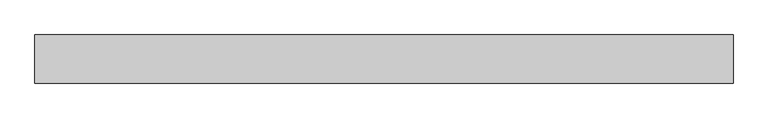
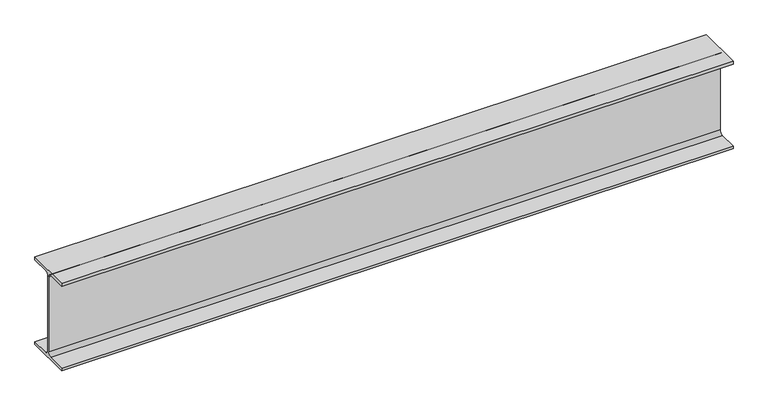
"""IFC4 building model written with IfcOpenShell, lengths in millimetres: beam geometry, 0912_Steel Framing_H-KSD3502 : H_SB_ASB_H-350x175x7x11."""

import ifcopenshell
import ifcopenshell.guid

model = None  # the IFC model being written
_history = None  # IfcOwnerHistory: only IFC2X3 demands one
_inside = {}  # id of a spatial element -> (the spatial element, [elements in it])
_under = {}  # id of a project, library or spatial element -> (it, [spatial elements below it])
_declared = {}  # id of a project -> (the project, [libraries it declares])
_typed = {}  # id of a type object -> (the type object, [elements of that type])
_made_of = {}  # id of a material, layer set ... -> (it, [elements and type objects made of it])


def new_model(schema):
    """Start an empty IFC model of exactly this schema.

    Asked for "IFC4X3", IfcOpenShell would pick the latest addendum, in which some entities
    have other attributes; the version numbers below select the first issue.
    IFC2X3 requires an IfcOwnerHistory on every rooted entity: one is made here for all.
    """
    global model, _history
    if schema == "IFC4X3":
        model = ifcopenshell.file(schema_version=(4, 3, 0, 0))
    else:
        model = ifcopenshell.file(schema=schema)
    _inside.clear()
    _under.clear()
    _declared.clear()
    _typed.clear()
    _made_of.clear()
    _history = None
    if model.schema == "IFC2X3":
        org = make("IfcOrganization", Name="unknown")
        user = make(
            "IfcPersonAndOrganization",
            ThePerson=make("IfcPerson", FamilyName="unknown"),
            TheOrganization=org,
        )
        app = make(
            "IfcApplication",
            ApplicationDeveloper=org,
            Version="unknown",
            ApplicationFullName="unknown",
            ApplicationIdentifier="unknown",
        )
        _history = make(
            "IfcOwnerHistory",
            OwningUser=user,
            OwningApplication=app,
            ChangeAction="ADDED",
            CreationDate=0,
        )
    return model


def make(cls, **values):
    """One entity of the class cls with the attributes given. An attribute that is None is left unset."""
    return model.create_entity(
        cls, **{name: value for name, value in values.items() if value is not None}
    )


def rooted(cls, **values):
    """An entity with a GlobalId (a new one), such as an element, a storey or a relation."""
    return make(cls, GlobalId=ifcopenshell.guid.new(), OwnerHistory=_history, **values)


def si_unit(unit_type, name, prefix=None):
    """IfcSIUnit, for example si_unit("LENGTHUNIT", "METRE", prefix="MILLI")."""
    return make("IfcSIUnit", UnitType=unit_type, Prefix=prefix, Name=name)


def assignment(units):
    """IfcUnitAssignment: the units of a project."""
    return None if units is None else make("IfcUnitAssignment", Units=units)


def point(xyz):
    """IfcCartesianPoint."""
    return None if xyz is None else make("IfcCartesianPoint", Coordinates=xyz)


def direction(xyz):
    """IfcDirection."""
    return None if xyz is None else make("IfcDirection", DirectionRatios=xyz)


def frame(location, z_axis=None, x_axis=None):
    """IfcAxis2Placement3D, a coordinate frame: its origin and axes. An axis left out is left unset."""
    return make(
        "IfcAxis2Placement3D",
        Location=point(location),
        Axis=direction(z_axis),
        RefDirection=direction(x_axis),
    )


def frame_2d(location, x_axis=None):
    """IfcAxis2Placement2D, a coordinate frame in the plane: its origin and x axis."""
    return make(
        "IfcAxis2Placement2D", Location=point(location), RefDirection=direction(x_axis)
    )


def origin():
    """The frame at (0, 0, 0) with its axes left unset."""
    return frame((0.0, 0.0, 0.0))


def place(relative_to, where):
    """IfcLocalPlacement: puts the frame where relative to a parent placement (None: the world)."""
    return make(
        "IfcLocalPlacement", PlacementRelTo=relative_to, RelativePlacement=where
    )


def context(
    kind, dimensions, precision=None, world=None, true_north=None, identifier=None
):
    """IfcGeometricRepresentationContext, for example the 3D "Model" context."""
    return make(
        "IfcGeometricRepresentationContext",
        ContextIdentifier=identifier,
        ContextType=kind,
        CoordinateSpaceDimension=dimensions,
        Precision=precision,
        WorldCoordinateSystem=world,
        TrueNorth=true_north,
    )


def project(units=None, contexts=None):
    """IfcProject with its units and contexts."""
    return rooted(
        "IfcProject",
        Name="project",
        RepresentationContexts=contexts,
        UnitsInContext=assignment(units),
    )


def spatial(cls, under=None, at=None, **own):
    """A site, building, storey or space (cls), placed at a placement, below another one or the project."""
    s = rooted(cls, ObjectPlacement=at, **own)
    if under is not None:
        _under.setdefault(under.id(), (under, []))[1].append(s)
    return s


def polyline(points):
    """IfcPolyline through the points."""
    return make("IfcPolyline", Points=[point(p) for p in points])


def circle_curve(where, radius):
    """IfcCircle in the frame where."""
    return make("IfcCircle", Position=where, Radius=radius)


def trimmed(basis, trim1, trim2, sense, master):
    """IfcTrimmedCurve: the piece of a basis curve between two trims."""
    return make(
        "IfcTrimmedCurve",
        BasisCurve=basis,
        Trim1=trim1,
        Trim2=trim2,
        SenseAgreement=sense,
        MasterRepresentation=master,
    )


def segment(curve, same_sense, transition):
    """IfcCompositeCurveSegment."""
    return make(
        "IfcCompositeCurveSegment",
        Transition=transition,
        SameSense=same_sense,
        ParentCurve=curve,
    )


def composite_curve(segments, self_intersect=None):
    """IfcCompositeCurve: segments joined end to end."""
    return make("IfcCompositeCurve", Segments=segments, SelfIntersect=self_intersect)


def outline(outer, holes=None, kind="AREA"):
    """IfcArbitraryClosedProfileDef: a profile drawn as a closed curve; with holes, ...WithVoids."""
    if holes is None:
        return make("IfcArbitraryClosedProfileDef", ProfileType=kind, OuterCurve=outer)
    return make(
        "IfcArbitraryProfileDefWithVoids",
        ProfileType=kind,
        OuterCurve=outer,
        InnerCurves=holes,
    )


def extrude(swept, where, along, depth):
    """IfcExtrudedAreaSolid: the profile swept, set in the frame where, extruded along a direction by depth."""
    return make(
        "IfcExtrudedAreaSolid",
        SweptArea=swept,
        Position=where,
        ExtrudedDirection=direction(along),
        Depth=depth,
    )


def shape(context_of_items, identifier, shape_type, items):
    """IfcShapeRepresentation: the items that make up one representation, for example the "Body"."""
    return make(
        "IfcShapeRepresentation",
        ContextOfItems=context_of_items,
        RepresentationIdentifier=identifier,
        RepresentationType=shape_type,
        Items=items,
    )


def source(mapping_origin, context_of_items, identifier, shape_type, items):
    """IfcRepresentationMap: a shape defined once, which mapped items show again and again."""
    return make(
        "IfcRepresentationMap",
        MappingOrigin=mapping_origin,
        MappedRepresentation=shape(context_of_items, identifier, shape_type, items),
    )


def transform(
    local_origin,
    x_axis=None,
    y_axis=None,
    z_axis=None,
    scale=None,
    scale2=None,
    scale3=None,
    uniform=True,
):
    """IfcCartesianTransformationOperator3D, or its non-uniform kind. x_axis, y_axis, z_axis: its Axis1, 2, 3."""
    if uniform:
        return make(
            "IfcCartesianTransformationOperator3D",
            Axis1=direction(x_axis),
            Axis2=direction(y_axis),
            LocalOrigin=point(local_origin),
            Scale=scale,
            Axis3=direction(z_axis),
        )
    return make(
        "IfcCartesianTransformationOperator3DnonUniform",
        Axis1=direction(x_axis),
        Axis2=direction(y_axis),
        LocalOrigin=point(local_origin),
        Scale=scale,
        Axis3=direction(z_axis),
        Scale2=scale2,
        Scale3=scale3,
    )


def mapped(mapping_source, mapping_target):
    """IfcMappedItem: shows the shape of a source again, moved by a transform."""
    return make(
        "IfcMappedItem", MappingSource=mapping_source, MappingTarget=mapping_target
    )


def made_of(thing, what):
    """Note that an element or type object is made of a material, layer set ...; save() writes the relation."""
    if what is not None:
        _made_of.setdefault(what.id(), (what, []))[1].append(thing)
    return thing


def element(
    cls,
    number,
    at=None,
    inside=None,
    cuts=None,
    type_object=None,
    material=None,
    context=None,
    identifier="Body",
    shape_type=None,
    held_by="IfcProductDefinitionShape",
    body=None,
    shapes=None,
    **own,
):
    """One element of the class cls, such as IfcWall. Its Tag is "e" and its number.

    at: its placement. inside: the storey or other place that contains it. cuts: it is an
    opening in that element (IfcRelVoidsElement). A single representation is given by context,
    identifier, shape_type and body (its items); several are given by shapes. held_by: the class
    of the entity that holds the representations. save() writes the other relations.
    """
    e = rooted(cls, Tag="e%d" % number, ObjectPlacement=at, **own)
    if body is not None:
        shapes = [shape(context, identifier, shape_type, body)]
    if shapes is not None:
        e.Representation = make(held_by, Representations=shapes)
    if inside is not None:
        _inside.setdefault(inside.id(), (inside, []))[1].append(e)
    if cuts is not None:
        rooted(
            "IfcRelVoidsElement", RelatingBuildingElement=cuts, RelatedOpeningElement=e
        )
    if type_object is not None:
        _typed.setdefault(type_object.id(), (type_object, []))[1].append(e)
    return made_of(e, material)


def aggregate(whole, parts):
    """IfcRelAggregates: a whole, such as a stair, and the parts it consists of."""
    return rooted("IfcRelAggregates", RelatingObject=whole, RelatedObjects=parts)


def save(model, path):
    """Write the relations noted so far, then the file.

    IfcRelAggregates (storeys below a building ...), IfcRelContainedInSpatialStructure (elements
    in a storey), IfcRelDefinesByType, IfcRelAssociatesMaterial and IfcRelDeclares: one each for
    every whole, place, type object, material and project.
    """
    for whole, parts in _under.values():
        aggregate(whole, parts)
    for where, things in _inside.values():
        rooted(
            "IfcRelContainedInSpatialStructure",
            RelatedElements=things,
            RelatingStructure=where,
        )
    for kind, things in _typed.values():
        rooted("IfcRelDefinesByType", RelatedObjects=things, RelatingType=kind)
    for what, things in _made_of.values():
        rooted("IfcRelAssociatesMaterial", RelatedObjects=things, RelatingMaterial=what)
    for by, libraries in _declared.values():
        rooted("IfcRelDeclares", RelatingContext=by, RelatedDefinitions=libraries)
    model.write(path)


def beam_0f635493(model_context):
    return source(origin(), model_context, "Body", "SweptSolid", [
        extrude(outline(composite_curve([segment(polyline([(87.5, -164.0), (87.5, -175.0), (-87.5, -175.0), (-87.5, -164.0), (-17.5, -164.0)]), True, "CONTINUOUS"), segment(trimmed(circle_curve(frame_2d((-17.5, -150.0)), 14.0), [point((-17.5, -164.0))], [point((-3.5, -150.0))], True, "CARTESIAN"), True, "CONTINUOUS"), segment(polyline([(-3.5, -150.0), (-3.5, 150.0)]), True, "CONTINUOUS"), segment(trimmed(circle_curve(frame_2d((-17.5, 150.0)), 14.0), [point((-3.5, 150.0))], [point((-17.5, 164.0))], True, "CARTESIAN"), True, "CONTINUOUS"), segment(polyline([(-17.5, 164.0), (-87.5, 164.0), (-87.5, 175.0), (87.5, 175.0), (87.5, 164.0), (17.5, 164.0)]), True, "CONTINUOUS"), segment(trimmed(circle_curve(frame_2d((17.5, 150.0)), 14.0), [point((17.5, 164.0))], [point((3.5, 150.0))], True, "CARTESIAN"), True, "CONTINUOUS"), segment(polyline([(3.5, 150.0), (3.5, -150.0)]), True, "CONTINUOUS"), segment(trimmed(circle_curve(frame_2d((17.5, -150.0)), 14.0), [point((3.5, -150.0))], [point((17.5, -164.0))], True, "CARTESIAN"), True, "CONTINUOUS"), segment(polyline([(17.5, -164.0), (87.5, -164.0)]), True, "CONTINUOUS")], self_intersect=False)), frame((-1295.7739051, 0.0, 0.0), z_axis=(1.0, 0.0, 0.0), x_axis=(0.0, 1.0, 0.0)), (0.0, 0.0, 1.0), 2540.0189947),
    ])


if __name__ == "__main__":
    model = new_model("IFC4")
    model_context = context("Model", 3, world=origin())
    ifc_project = project(units=[si_unit("LENGTHUNIT", "METRE", prefix="MILLI")], contexts=[model_context])
    site = spatial("IfcSite", under=ifc_project)
    building = spatial("IfcBuilding", under=site)
    placement = place(None, origin())
    beam_shape = beam_0f635493(model_context)
    element("IfcBeam", 1, ObjectType="0912_Steel Framing_H-KSD3502 : H_SB_ASB_H-350x175x7x11", at=placement, inside=building, context=model_context, shape_type="MappedRepresentation", body=[
        mapped(beam_shape, transform((0.0, 0.0, 0.0), x_axis=(1.0, 0.0, 0.0), y_axis=(0.0, 1.0, 0.0), z_axis=(0.0, 0.0, 1.0))),
    ])
    save(model, "model.ifc")

# Revit data of these elements
# Type "0912_Steel Framing_H-KSD3502 : H_SB_ASB_H-350x175x7x11"
#   H_WM Code_1 = "S01AA002-00001 | Main Steel Structure Fabrication Work | Shelter/Building | Medium Steel - Standard (90KG/M>Weight≥30KG/M) | Material: (   )"
#   H_WM Code_2 = "S03AA028-00001 | Main Steel Structure Erection Work | Shelter/Building | Medium Steel (90KG/M>Weight≥30KG/M) | Material: (   )"
#   H_WM Code_3 = "S01AA010-00001 | Main Steel Structure Fabrication Work | Shelter/Building | Steel Painting/Coating | for Non-Fireproofed Steel Surface, Surface Preparation, Primer, Second & Final Coat | Material: (   )"
#   H_Q'ty Cal Type Tag = "SB-Q2"
#   Width = 17.5 cm
#   Web Thickness = 0.7 cm
#   Web Fillet = 1.4 cm
#   Warping Constant = 282000.0 cm⁶
#   W = 0
#   Torsional Moment of Inertia = 19.4042 cm⁴
#   Section Area = 63.14 cm²
#   Plastic Modulus weak axis = 174.0 cm³
#   Plastic Modulus strong axis = 868.0 cm³
#   Perimeter = 1.36 m²/m
#   Nominal Weight = 49.60 kgf/m
#   Moment of Inertia weak axis = 984.00 cm⁴
#   Moment of Inertia strong axis = 13600.00 cm⁴
#   Height = 35.0 cm
#   Flange Thickness = 1.1 cm
#   Elastic Modulus weak axis = 112.0 cm³
#   Elastic Modulus strong axis = 775.0 cm³
#   Centroid Vertical = 17.5 cm
#   Centroid Horizontal = 8.75 cm
#   Ix = 136000000
#   Length [instance default] = 1.5240 m
#   Zx = 868000
#   b = 0.1750 m
#   h = 0.3500 m
#   r = 0.0140 m
#   s = 0.0070 m
#   t = 0.0110 m
#   A = 0.006314 m²
#   Structural Material [instance default] = Steel, 45-345
#   Assembly Code = ""
# Element 1 (IfcBeam, "0912_Steel Framing_H-KSD3502 : H_SB_ASB_H-350x175x7x11")
#   Structural Material = none
# Materials
#   "Steel, 45-345": class "Metal", colour RGB 189 187 185, transparency 0, Description = "Steel 345 MPa", Cost = 0
